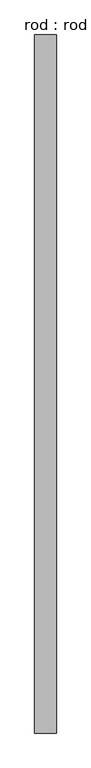
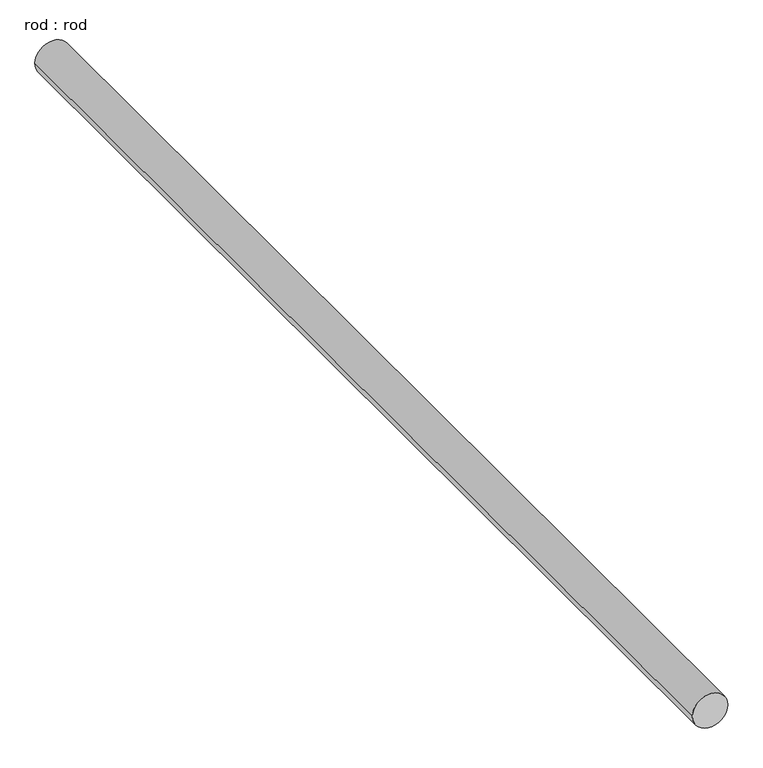
"""IFC4 building model written with IfcOpenShell, lengths in millimetres: proxy geometry, rod : rod."""

from ifc_helpers import new_model, si_unit, point, frame, frame_2d, origin, place, context, project, spatial, circle_curve, trimmed, segment, composite_curve, outline, extrude, source, transform, mapped, element, save


def rod_rod_1a174f2f(model_context):
    return source(origin(), model_context, "Body", "SweptSolid", [
        extrude(outline(composite_curve([segment(trimmed(circle_curve(frame_2d((0.0108462, 0.0)), 200.0), [point((0.0108462, 200.0))], [point((0.0108462, -200.0))], False, "CARTESIAN"), True, "CONTINUOUS"), segment(trimmed(circle_curve(frame_2d((0.0108462, 0.0)), 200.0), [point((0.0108462, -200.0))], [point((0.0108462, 200.0))], False, "CARTESIAN"), True, "CONTINUOUS")], self_intersect=False)), frame((0.0, -2359.5899698, 0.0), z_axis=(0.0, 1.0, 0.0), x_axis=(0.0, 0.0, 1.0)), (0.0, 0.0, 1.0), 12904.6371702),
    ])


if __name__ == "__main__":
    model = new_model("IFC4")
    model_context = context("Model", 3, world=origin())
    ifc_project = project(units=[si_unit("LENGTHUNIT", "METRE", prefix="MILLI")], contexts=[model_context])
    site = spatial("IfcSite", under=ifc_project)
    building = spatial("IfcBuilding", under=site)
    placement = place(None, origin())
    rod_rod_shape = rod_rod_1a174f2f(model_context)
    element("IfcBuildingElementProxy", 1, Name="rod : rod", ObjectType="rod : rod", at=placement, inside=building, context=model_context, shape_type="MappedRepresentation", body=[
        mapped(rod_rod_shape, transform((0.0, 0.0, 0.0), x_axis=(1.0, 0.0, 0.0), y_axis=(0.0, 1.0, 0.0), z_axis=(0.0, 0.0, 1.0))),
    ])
    save(model, "model.ifc")

# Revit data of these elements
# Type "rod : rod"
#   Default Elevation = 0
